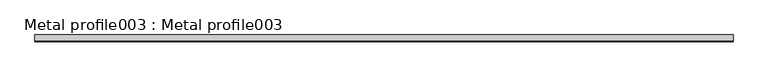
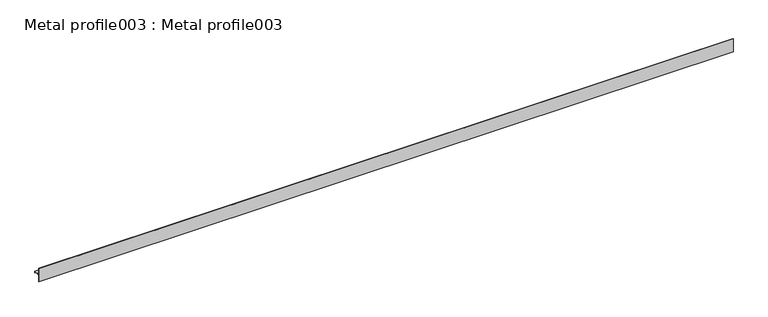
"""IFC4 building model written with IfcOpenShell, lengths in millimetres: proxy geometry, Metal profile003 : Metal profile003."""

import ifcopenshell
import ifcopenshell.guid

model = None  # the IFC model being written
_history = None  # IfcOwnerHistory: only IFC2X3 demands one
_inside = {}  # id of a spatial element -> (the spatial element, [elements in it])
_under = {}  # id of a project, library or spatial element -> (it, [spatial elements below it])
_declared = {}  # id of a project -> (the project, [libraries it declares])
_typed = {}  # id of a type object -> (the type object, [elements of that type])
_made_of = {}  # id of a material, layer set ... -> (it, [elements and type objects made of it])


def new_model(schema):
    """Start an empty IFC model of exactly this schema.

    Asked for "IFC4X3", IfcOpenShell would pick the latest addendum, in which some entities
    have other attributes; the version numbers below select the first issue.
    IFC2X3 requires an IfcOwnerHistory on every rooted entity: one is made here for all.
    """
    global model, _history
    if schema == "IFC4X3":
        model = ifcopenshell.file(schema_version=(4, 3, 0, 0))
    else:
        model = ifcopenshell.file(schema=schema)
    _inside.clear()
    _under.clear()
    _declared.clear()
    _typed.clear()
    _made_of.clear()
    _history = None
    if model.schema == "IFC2X3":
        org = make("IfcOrganization", Name="unknown")
        user = make(
            "IfcPersonAndOrganization",
            ThePerson=make("IfcPerson", FamilyName="unknown"),
            TheOrganization=org,
        )
        app = make(
            "IfcApplication",
            ApplicationDeveloper=org,
            Version="unknown",
            ApplicationFullName="unknown",
            ApplicationIdentifier="unknown",
        )
        _history = make(
            "IfcOwnerHistory",
            OwningUser=user,
            OwningApplication=app,
            ChangeAction="ADDED",
            CreationDate=0,
        )
    return model


def make(cls, **values):
    """One entity of the class cls with the attributes given. An attribute that is None is left unset."""
    return model.create_entity(
        cls, **{name: value for name, value in values.items() if value is not None}
    )


def rooted(cls, **values):
    """An entity with a GlobalId (a new one), such as an element, a storey or a relation."""
    return make(cls, GlobalId=ifcopenshell.guid.new(), OwnerHistory=_history, **values)


def si_unit(unit_type, name, prefix=None):
    """IfcSIUnit, for example si_unit("LENGTHUNIT", "METRE", prefix="MILLI")."""
    return make("IfcSIUnit", UnitType=unit_type, Prefix=prefix, Name=name)


def assignment(units):
    """IfcUnitAssignment: the units of a project."""
    return None if units is None else make("IfcUnitAssignment", Units=units)


def point(xyz):
    """IfcCartesianPoint."""
    return None if xyz is None else make("IfcCartesianPoint", Coordinates=xyz)


def direction(xyz):
    """IfcDirection."""
    return None if xyz is None else make("IfcDirection", DirectionRatios=xyz)


def frame(location, z_axis=None, x_axis=None):
    """IfcAxis2Placement3D, a coordinate frame: its origin and axes. An axis left out is left unset."""
    return make(
        "IfcAxis2Placement3D",
        Location=point(location),
        Axis=direction(z_axis),
        RefDirection=direction(x_axis),
    )


def origin():
    """The frame at (0, 0, 0) with its axes left unset."""
    return frame((0.0, 0.0, 0.0))


def place(relative_to, where):
    """IfcLocalPlacement: puts the frame where relative to a parent placement (None: the world)."""
    return make(
        "IfcLocalPlacement", PlacementRelTo=relative_to, RelativePlacement=where
    )


def context(
    kind, dimensions, precision=None, world=None, true_north=None, identifier=None
):
    """IfcGeometricRepresentationContext, for example the 3D "Model" context."""
    return make(
        "IfcGeometricRepresentationContext",
        ContextIdentifier=identifier,
        ContextType=kind,
        CoordinateSpaceDimension=dimensions,
        Precision=precision,
        WorldCoordinateSystem=world,
        TrueNorth=true_north,
    )


def project(units=None, contexts=None):
    """IfcProject with its units and contexts."""
    return rooted(
        "IfcProject",
        Name="project",
        RepresentationContexts=contexts,
        UnitsInContext=assignment(units),
    )


def spatial(cls, under=None, at=None, **own):
    """A site, building, storey or space (cls), placed at a placement, below another one or the project."""
    s = rooted(cls, ObjectPlacement=at, **own)
    if under is not None:
        _under.setdefault(under.id(), (under, []))[1].append(s)
    return s


def polyline(points):
    """IfcPolyline through the points."""
    return make("IfcPolyline", Points=[point(p) for p in points])


def outline(outer, holes=None, kind="AREA"):
    """IfcArbitraryClosedProfileDef: a profile drawn as a closed curve; with holes, ...WithVoids."""
    if holes is None:
        return make("IfcArbitraryClosedProfileDef", ProfileType=kind, OuterCurve=outer)
    return make(
        "IfcArbitraryProfileDefWithVoids",
        ProfileType=kind,
        OuterCurve=outer,
        InnerCurves=holes,
    )


def extrude(swept, where, along, depth):
    """IfcExtrudedAreaSolid: the profile swept, set in the frame where, extruded along a direction by depth."""
    return make(
        "IfcExtrudedAreaSolid",
        SweptArea=swept,
        Position=where,
        ExtrudedDirection=direction(along),
        Depth=depth,
    )


def shape(context_of_items, identifier, shape_type, items):
    """IfcShapeRepresentation: the items that make up one representation, for example the "Body"."""
    return make(
        "IfcShapeRepresentation",
        ContextOfItems=context_of_items,
        RepresentationIdentifier=identifier,
        RepresentationType=shape_type,
        Items=items,
    )


def source(mapping_origin, context_of_items, identifier, shape_type, items):
    """IfcRepresentationMap: a shape defined once, which mapped items show again and again."""
    return make(
        "IfcRepresentationMap",
        MappingOrigin=mapping_origin,
        MappedRepresentation=shape(context_of_items, identifier, shape_type, items),
    )


def transform(
    local_origin,
    x_axis=None,
    y_axis=None,
    z_axis=None,
    scale=None,
    scale2=None,
    scale3=None,
    uniform=True,
):
    """IfcCartesianTransformationOperator3D, or its non-uniform kind. x_axis, y_axis, z_axis: its Axis1, 2, 3."""
    if uniform:
        return make(
            "IfcCartesianTransformationOperator3D",
            Axis1=direction(x_axis),
            Axis2=direction(y_axis),
            LocalOrigin=point(local_origin),
            Scale=scale,
            Axis3=direction(z_axis),
        )
    return make(
        "IfcCartesianTransformationOperator3DnonUniform",
        Axis1=direction(x_axis),
        Axis2=direction(y_axis),
        LocalOrigin=point(local_origin),
        Scale=scale,
        Axis3=direction(z_axis),
        Scale2=scale2,
        Scale3=scale3,
    )


def mapped(mapping_source, mapping_target):
    """IfcMappedItem: shows the shape of a source again, moved by a transform."""
    return make(
        "IfcMappedItem", MappingSource=mapping_source, MappingTarget=mapping_target
    )


def made_of(thing, what):
    """Note that an element or type object is made of a material, layer set ...; save() writes the relation."""
    if what is not None:
        _made_of.setdefault(what.id(), (what, []))[1].append(thing)
    return thing


def element(
    cls,
    number,
    at=None,
    inside=None,
    cuts=None,
    type_object=None,
    material=None,
    context=None,
    identifier="Body",
    shape_type=None,
    held_by="IfcProductDefinitionShape",
    body=None,
    shapes=None,
    **own,
):
    """One element of the class cls, such as IfcWall. Its Tag is "e" and its number.

    at: its placement. inside: the storey or other place that contains it. cuts: it is an
    opening in that element (IfcRelVoidsElement). A single representation is given by context,
    identifier, shape_type and body (its items); several are given by shapes. held_by: the class
    of the entity that holds the representations. save() writes the other relations.
    """
    e = rooted(cls, Tag="e%d" % number, ObjectPlacement=at, **own)
    if body is not None:
        shapes = [shape(context, identifier, shape_type, body)]
    if shapes is not None:
        e.Representation = make(held_by, Representations=shapes)
    if inside is not None:
        _inside.setdefault(inside.id(), (inside, []))[1].append(e)
    if cuts is not None:
        rooted(
            "IfcRelVoidsElement", RelatingBuildingElement=cuts, RelatedOpeningElement=e
        )
    if type_object is not None:
        _typed.setdefault(type_object.id(), (type_object, []))[1].append(e)
    return made_of(e, material)


def aggregate(whole, parts):
    """IfcRelAggregates: a whole, such as a stair, and the parts it consists of."""
    return rooted("IfcRelAggregates", RelatingObject=whole, RelatedObjects=parts)


def save(model, path):
    """Write the relations noted so far, then the file.

    IfcRelAggregates (storeys below a building ...), IfcRelContainedInSpatialStructure (elements
    in a storey), IfcRelDefinesByType, IfcRelAssociatesMaterial and IfcRelDeclares: one each for
    every whole, place, type object, material and project.
    """
    for whole, parts in _under.values():
        aggregate(whole, parts)
    for where, things in _inside.values():
        rooted(
            "IfcRelContainedInSpatialStructure",
            RelatedElements=things,
            RelatingStructure=where,
        )
    for kind, things in _typed.values():
        rooted("IfcRelDefinesByType", RelatedObjects=things, RelatingType=kind)
    for what, things in _made_of.values():
        rooted("IfcRelAssociatesMaterial", RelatedObjects=things, RelatingMaterial=what)
    for by, libraries in _declared.values():
        rooted("IfcRelDeclares", RelatingContext=by, RelatedDefinitions=libraries)
    model.write(path)


def metal_profile003_metal_profile003_84f21a9e(model_context):
    return source(origin(), model_context, "Body", "SweptSolid", [
        extrude(outline(polyline([(9773.5175834, 37481.0682813), (9756.5536354, 37481.0682813), (9756.5536354, 37462.0182812), (9755.2836354, 37462.0182812), (9755.2836354, 37501.3882813), (9756.5536354, 37501.3882813), (9756.5536354, 37482.3382813), (9774.7875834, 37482.3382813), (9774.7875834, 37477.5884813), (9773.5175834, 37477.5884813), (9773.5175834, 37481.0682813)])), frame((3694.2883192, 0.0, 0.0), z_axis=(1.0, 0.0, 0.0), x_axis=(0.0, 1.0, 0.0)), (0.0, 0.0, 1.0), 2000.0),
    ])


if __name__ == "__main__":
    model = new_model("IFC4")
    model_context = context("Model", 3, world=origin())
    ifc_project = project(units=[si_unit("LENGTHUNIT", "METRE", prefix="MILLI")], contexts=[model_context])
    site = spatial("IfcSite", under=ifc_project)
    building = spatial("IfcBuilding", under=site)
    placement = place(None, origin())
    metal_profile003_metal_profile003_shape = metal_profile003_metal_profile003_84f21a9e(model_context)
    element("IfcBuildingElementProxy", 1, Name="Metal profile003 : Metal profile003", ObjectType="Metal profile003 : Metal profile003", at=placement, inside=building, context=model_context, shape_type="MappedRepresentation", body=[
        mapped(metal_profile003_metal_profile003_shape, transform((0.0, 0.0, 0.0), x_axis=(1.0, 0.0, 0.0), y_axis=(0.0, 1.0, 0.0), z_axis=(0.0, 0.0, 1.0))),
    ])
    save(model, "model.ifc")

# Revit data of these elements
# Type "Metal profile003 : Metal profile003"
#   NameOverride = "Metal profile003"
# Element 1 (IfcBuildingElementProxy, "Metal profile003 : Metal profile003")
#   Materials on its faces: "16 GA. COPPER VENTED T REVEAL BEAD"
# Materials
#   "16 GA. COPPER VENTED T REVEAL BEAD": class "Unassigned", colour RGB 255 227 10, transparency 0
